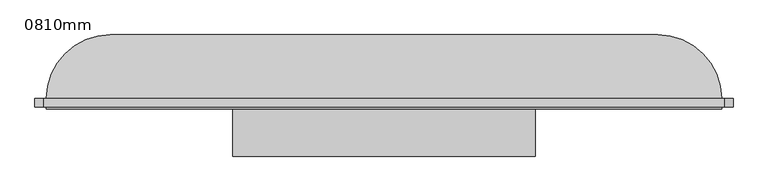
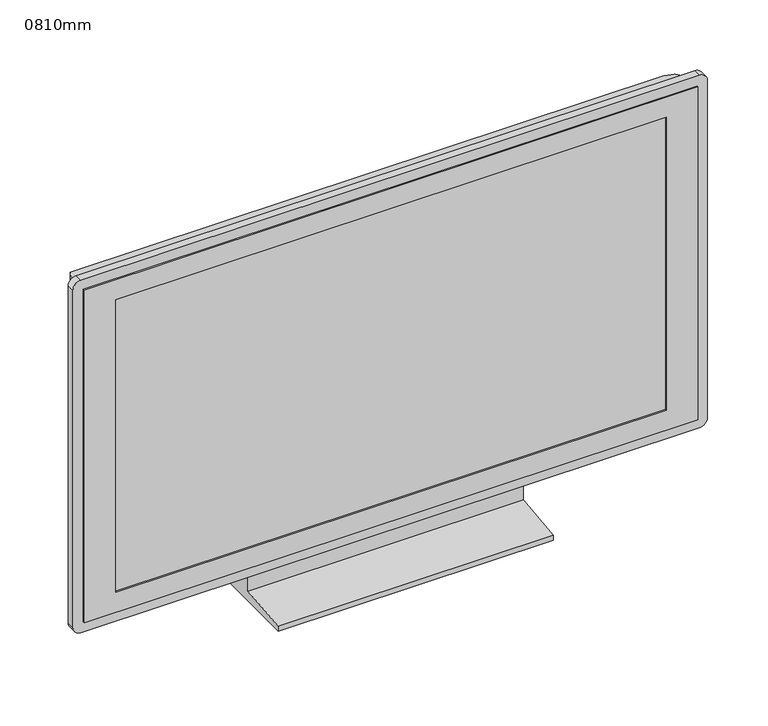
"""IFC4 building model written with IfcOpenShell, lengths in millimetres: furniture geometry, M_TV - Flat Screen : 0810mm."""

import ifcopenshell
import ifcopenshell.guid

model = None  # the IFC model being written
_history = None  # IfcOwnerHistory: only IFC2X3 demands one
_inside = {}  # id of a spatial element -> (the spatial element, [elements in it])
_under = {}  # id of a project, library or spatial element -> (it, [spatial elements below it])
_declared = {}  # id of a project -> (the project, [libraries it declares])
_typed = {}  # id of a type object -> (the type object, [elements of that type])
_made_of = {}  # id of a material, layer set ... -> (it, [elements and type objects made of it])


def new_model(schema):
    """Start an empty IFC model of exactly this schema.

    Asked for "IFC4X3", IfcOpenShell would pick the latest addendum, in which some entities
    have other attributes; the version numbers below select the first issue.
    IFC2X3 requires an IfcOwnerHistory on every rooted entity: one is made here for all.
    """
    global model, _history
    if schema == "IFC4X3":
        model = ifcopenshell.file(schema_version=(4, 3, 0, 0))
    else:
        model = ifcopenshell.file(schema=schema)
    _inside.clear()
    _under.clear()
    _declared.clear()
    _typed.clear()
    _made_of.clear()
    _history = None
    if model.schema == "IFC2X3":
        org = make("IfcOrganization", Name="unknown")
        user = make(
            "IfcPersonAndOrganization",
            ThePerson=make("IfcPerson", FamilyName="unknown"),
            TheOrganization=org,
        )
        app = make(
            "IfcApplication",
            ApplicationDeveloper=org,
            Version="unknown",
            ApplicationFullName="unknown",
            ApplicationIdentifier="unknown",
        )
        _history = make(
            "IfcOwnerHistory",
            OwningUser=user,
            OwningApplication=app,
            ChangeAction="ADDED",
            CreationDate=0,
        )
    return model


def make(cls, **values):
    """One entity of the class cls with the attributes given. An attribute that is None is left unset."""
    return model.create_entity(
        cls, **{name: value for name, value in values.items() if value is not None}
    )


def rooted(cls, **values):
    """An entity with a GlobalId (a new one), such as an element, a storey or a relation."""
    return make(cls, GlobalId=ifcopenshell.guid.new(), OwnerHistory=_history, **values)


def si_unit(unit_type, name, prefix=None):
    """IfcSIUnit, for example si_unit("LENGTHUNIT", "METRE", prefix="MILLI")."""
    return make("IfcSIUnit", UnitType=unit_type, Prefix=prefix, Name=name)


def assignment(units):
    """IfcUnitAssignment: the units of a project."""
    return None if units is None else make("IfcUnitAssignment", Units=units)


def point(xyz):
    """IfcCartesianPoint."""
    return None if xyz is None else make("IfcCartesianPoint", Coordinates=xyz)


def direction(xyz):
    """IfcDirection."""
    return None if xyz is None else make("IfcDirection", DirectionRatios=xyz)


def frame(location, z_axis=None, x_axis=None):
    """IfcAxis2Placement3D, a coordinate frame: its origin and axes. An axis left out is left unset."""
    return make(
        "IfcAxis2Placement3D",
        Location=point(location),
        Axis=direction(z_axis),
        RefDirection=direction(x_axis),
    )


def frame_2d(location, x_axis=None):
    """IfcAxis2Placement2D, a coordinate frame in the plane: its origin and x axis."""
    return make(
        "IfcAxis2Placement2D", Location=point(location), RefDirection=direction(x_axis)
    )


def origin():
    """The frame at (0, 0, 0) with its axes left unset."""
    return frame((0.0, 0.0, 0.0))


def place(relative_to, where):
    """IfcLocalPlacement: puts the frame where relative to a parent placement (None: the world)."""
    return make(
        "IfcLocalPlacement", PlacementRelTo=relative_to, RelativePlacement=where
    )


def context(
    kind, dimensions, precision=None, world=None, true_north=None, identifier=None
):
    """IfcGeometricRepresentationContext, for example the 3D "Model" context."""
    return make(
        "IfcGeometricRepresentationContext",
        ContextIdentifier=identifier,
        ContextType=kind,
        CoordinateSpaceDimension=dimensions,
        Precision=precision,
        WorldCoordinateSystem=world,
        TrueNorth=true_north,
    )


def project(units=None, contexts=None):
    """IfcProject with its units and contexts."""
    return rooted(
        "IfcProject",
        Name="project",
        RepresentationContexts=contexts,
        UnitsInContext=assignment(units),
    )


def spatial(cls, under=None, at=None, **own):
    """A site, building, storey or space (cls), placed at a placement, below another one or the project."""
    s = rooted(cls, ObjectPlacement=at, **own)
    if under is not None:
        _under.setdefault(under.id(), (under, []))[1].append(s)
    return s


def polyline(points):
    """IfcPolyline through the points."""
    return make("IfcPolyline", Points=[point(p) for p in points])


def circle_curve(where, radius):
    """IfcCircle in the frame where."""
    return make("IfcCircle", Position=where, Radius=radius)


def ellipse_curve(where, semi_axis1, semi_axis2):
    """IfcEllipse in the frame where."""
    return make(
        "IfcEllipse", Position=where, SemiAxis1=semi_axis1, SemiAxis2=semi_axis2
    )


def trimmed(basis, trim1, trim2, sense, master):
    """IfcTrimmedCurve: the piece of a basis curve between two trims."""
    return make(
        "IfcTrimmedCurve",
        BasisCurve=basis,
        Trim1=trim1,
        Trim2=trim2,
        SenseAgreement=sense,
        MasterRepresentation=master,
    )


def segment(curve, same_sense, transition):
    """IfcCompositeCurveSegment."""
    return make(
        "IfcCompositeCurveSegment",
        Transition=transition,
        SameSense=same_sense,
        ParentCurve=curve,
    )


def composite_curve(segments, self_intersect=None):
    """IfcCompositeCurve: segments joined end to end."""
    return make("IfcCompositeCurve", Segments=segments, SelfIntersect=self_intersect)


def outline(outer, holes=None, kind="AREA"):
    """IfcArbitraryClosedProfileDef: a profile drawn as a closed curve; with holes, ...WithVoids."""
    if holes is None:
        return make("IfcArbitraryClosedProfileDef", ProfileType=kind, OuterCurve=outer)
    return make(
        "IfcArbitraryProfileDefWithVoids",
        ProfileType=kind,
        OuterCurve=outer,
        InnerCurves=holes,
    )


def extrude(swept, where, along, depth):
    """IfcExtrudedAreaSolid: the profile swept, set in the frame where, extruded along a direction by depth."""
    return make(
        "IfcExtrudedAreaSolid",
        SweptArea=swept,
        Position=where,
        ExtrudedDirection=direction(along),
        Depth=depth,
    )


def faces_of(points, faces, orient=None, outer=None):
    """IfcFace entities. A face is a list of loops; a loop is a list of indices into points, from 0.

    orient and outer hold one flag for each loop. By default every Orientation is true, the
    first loop of a face is its IfcFaceOuterBound and the others are IfcFaceBound.
    """
    made = []
    for i, loops in enumerate(faces):
        bounds = []
        for j, loop in enumerate(loops):
            is_outer = j == 0 if outer is None else outer[i][j]
            bounds.append(
                make(
                    "IfcFaceOuterBound" if is_outer else "IfcFaceBound",
                    Bound=make("IfcPolyLoop", Polygon=[points[k] for k in loop]),
                    Orientation=True if orient is None else orient[i][j],
                )
            )
        made.append(make("IfcFace", Bounds=bounds))
    return made


def faceted_brep(points, faces, orient=None, outer=None, voids=None):
    """IfcFacetedBrep: a solid bounded by flat faces; with voids (closed shells), ...WithVoids."""
    shared = [point(p) for p in points]
    hull = make("IfcClosedShell", CfsFaces=faces_of(shared, faces, orient, outer))
    if voids is None:
        return make("IfcFacetedBrep", Outer=hull)
    return make(
        "IfcFacetedBrepWithVoids",
        Outer=hull,
        Voids=[
            make(cls, CfsFaces=faces_of(shared, fs, o, b)) for cls, fs, o, b in voids
        ],
    )


def shape(context_of_items, identifier, shape_type, items):
    """IfcShapeRepresentation: the items that make up one representation, for example the "Body"."""
    return make(
        "IfcShapeRepresentation",
        ContextOfItems=context_of_items,
        RepresentationIdentifier=identifier,
        RepresentationType=shape_type,
        Items=items,
    )


def source(mapping_origin, context_of_items, identifier, shape_type, items):
    """IfcRepresentationMap: a shape defined once, which mapped items show again and again."""
    return make(
        "IfcRepresentationMap",
        MappingOrigin=mapping_origin,
        MappedRepresentation=shape(context_of_items, identifier, shape_type, items),
    )


def transform(
    local_origin,
    x_axis=None,
    y_axis=None,
    z_axis=None,
    scale=None,
    scale2=None,
    scale3=None,
    uniform=True,
):
    """IfcCartesianTransformationOperator3D, or its non-uniform kind. x_axis, y_axis, z_axis: its Axis1, 2, 3."""
    if uniform:
        return make(
            "IfcCartesianTransformationOperator3D",
            Axis1=direction(x_axis),
            Axis2=direction(y_axis),
            LocalOrigin=point(local_origin),
            Scale=scale,
            Axis3=direction(z_axis),
        )
    return make(
        "IfcCartesianTransformationOperator3DnonUniform",
        Axis1=direction(x_axis),
        Axis2=direction(y_axis),
        LocalOrigin=point(local_origin),
        Scale=scale,
        Axis3=direction(z_axis),
        Scale2=scale2,
        Scale3=scale3,
    )


def mapped(mapping_source, mapping_target):
    """IfcMappedItem: shows the shape of a source again, moved by a transform."""
    return make(
        "IfcMappedItem", MappingSource=mapping_source, MappingTarget=mapping_target
    )


def made_of(thing, what):
    """Note that an element or type object is made of a material, layer set ...; save() writes the relation."""
    if what is not None:
        _made_of.setdefault(what.id(), (what, []))[1].append(thing)
    return thing


def element(
    cls,
    number,
    at=None,
    inside=None,
    cuts=None,
    type_object=None,
    material=None,
    context=None,
    identifier="Body",
    shape_type=None,
    held_by="IfcProductDefinitionShape",
    body=None,
    shapes=None,
    **own,
):
    """One element of the class cls, such as IfcWall. Its Tag is "e" and its number.

    at: its placement. inside: the storey or other place that contains it. cuts: it is an
    opening in that element (IfcRelVoidsElement). A single representation is given by context,
    identifier, shape_type and body (its items); several are given by shapes. held_by: the class
    of the entity that holds the representations. save() writes the other relations.
    """
    e = rooted(cls, Tag="e%d" % number, ObjectPlacement=at, **own)
    if body is not None:
        shapes = [shape(context, identifier, shape_type, body)]
    if shapes is not None:
        e.Representation = make(held_by, Representations=shapes)
    if inside is not None:
        _inside.setdefault(inside.id(), (inside, []))[1].append(e)
    if cuts is not None:
        rooted(
            "IfcRelVoidsElement", RelatingBuildingElement=cuts, RelatedOpeningElement=e
        )
    if type_object is not None:
        _typed.setdefault(type_object.id(), (type_object, []))[1].append(e)
    return made_of(e, material)


def aggregate(whole, parts):
    """IfcRelAggregates: a whole, such as a stair, and the parts it consists of."""
    return rooted("IfcRelAggregates", RelatingObject=whole, RelatedObjects=parts)


def save(model, path):
    """Write the relations noted so far, then the file.

    IfcRelAggregates (storeys below a building ...), IfcRelContainedInSpatialStructure (elements
    in a storey), IfcRelDefinesByType, IfcRelAssociatesMaterial and IfcRelDeclares: one each for
    every whole, place, type object, material and project.
    """
    for whole, parts in _under.values():
        aggregate(whole, parts)
    for where, things in _inside.values():
        rooted(
            "IfcRelContainedInSpatialStructure",
            RelatedElements=things,
            RelatingStructure=where,
        )
    for kind, things in _typed.values():
        rooted("IfcRelDefinesByType", RelatedObjects=things, RelatingType=kind)
    for what, things in _made_of.values():
        rooted("IfcRelAssociatesMaterial", RelatedObjects=things, RelatingMaterial=what)
    for by, libraries in _declared.values():
        rooted("IfcRelDeclares", RelatingContext=by, RelatedDefinitions=libraries)
    model.write(path)


def plane_surface(at):
    """IfcPlane: the flat surface through the origin of the frame at, square to its z axis."""
    return make("IfcPlane", Position=at)


def cylinder_surface(at, radius):
    """IfcCylindricalSurface: all points at the distance radius from the z axis of the frame at."""
    return make("IfcCylindricalSurface", Position=at, Radius=radius)


def advanced_brep(points, edges, surfaces, faces):
    """IfcAdvancedBrep: a solid bounded by faces that lie on surfaces and meet in shared edges.

    An edge is (start, end): straight between two places in points (the first is 0);
    or (start, end, curve); or (start, end, curve, False) where it runs against its curve.
    A face is (place in surfaces, loops), or (place, loops, False) where it looks against
    its surface's normal. A loop lists edges by number (the first is 1), with a minus sign
    where the edge is run from its end to its start. The first loop is the outer one.
    """
    corners = [point(p) for p in points]
    vertices = [make("IfcVertexPoint", VertexGeometry=c) for c in corners]
    made = []
    for start, end, *more in edges:
        made.append(
            make(
                "IfcEdgeCurve",
                EdgeStart=vertices[start],
                EdgeEnd=vertices[end],
                EdgeGeometry=more[0] if more else make("IfcPolyline", Points=[corners[start], corners[end]]),
                SameSense=more[1] if len(more) > 1 else True,
            )
        )
    hull = []
    for where, loops, *sense in faces:
        bounds = []
        for j, loop in enumerate(loops):
            ring = [make("IfcOrientedEdge", EdgeElement=made[abs(k) - 1], Orientation=k > 0) for k in loop]
            bounds.append(
                make(
                    "IfcFaceOuterBound" if j == 0 else "IfcFaceBound",
                    Bound=make("IfcEdgeLoop", EdgeList=ring),
                    Orientation=True,
                )
            )
        hull.append(make("IfcAdvancedFace", Bounds=bounds, FaceSurface=surfaces[where], SameSense=sense[0] if sense else True))
    return make("IfcAdvancedBrep", Outer=make("IfcClosedShell", CfsFaces=hull))


def furniture_0810mm_d9060323(model_context):
    return source(origin(), model_context, "Body", "SolidModel", [
        advanced_brep(
        [(-586.8783027, -51.4613764, 80.0), (578.9892744, -51.4613764, 80.0), (578.9892744, -51.4613764, 748.3544945), (-586.8783027, -51.4613764, 748.3544945), (468.9892744, 58.5386236, 80.0), (-476.8783027, 58.5386236, 80.0), (-476.8783027, 58.5386236, 638.3544945), (468.9892744, 58.5386236, 638.3544945)],
        [
            (0, 1),
            (1, 2),
            (2, 3),
            (3, 0),
            (4, 5),
            (5, 6),
            (6, 7),
            (7, 4),
            (0, 5, circle_curve(frame((-476.8783027, -51.4613764, 80.0), z_axis=(0.0, 0.0, -1.0), x_axis=(-1.0, 0.0, 0.0)), 110.0)),
            (4, 1, circle_curve(frame((468.9892744, -51.4613764, 80.0), z_axis=(0.0, 0.0, -1.0), x_axis=(1.0, 0.0, 0.0)), 110.0)),
            (7, 2, ellipse_curve(frame((468.9892744, -51.4613764, 638.3544945), z_axis=(0.7071067811865475, 0.0, -0.7071067811865475), x_axis=(0.7071067811865474, 0.0, 0.7071067811865476)), 155.5634919, 110.0)),
            (6, 3, ellipse_curve(frame((-476.8783027, -51.4613764, 638.3544945), z_axis=(0.7071067811865475, 0.0, 0.7071067811865476), x_axis=(-0.7071067811865476, 0.0, 0.7071067811865475)), 155.5634919, 110.0)),
        ],
        [
            plane_surface(frame((-586.8783027, -51.4613764, 748.3544945), z_axis=(0.0, -1.0, 0.0), x_axis=(-1.0, 0.0, 0.0))),
            plane_surface(frame((-586.8783027, 58.5386236, 748.3544945), z_axis=(0.0, 1.0, 0.0), x_axis=(1.0, 0.0, 0.0))),
            plane_surface(frame((-586.8783027, -51.4613764, 80.0), z_axis=(0.0, 0.0, -1.0), x_axis=(0.0, 1.0, 0.0))),
            cylinder_surface(frame((468.9892744, -51.4613764, 80.0), z_axis=(0.0, 0.0, 1.0), x_axis=(1.0, 0.0, 0.0)), 110.0),
            cylinder_surface(frame((578.9892744, -51.4613764, 638.3544945), z_axis=(-1.0, 0.0, 0.0), x_axis=(0.0, 0.0, 1.0)), 110.0),
            cylinder_surface(frame((-476.8783027, -51.4613764, 748.3544945), z_axis=(0.0, 0.0, -1.0), x_axis=(-1.0, 0.0, 0.0)), 110.0),
        ],
        [
            (0, [[1, 2, 3, 4]]),
            (1, [[5, 6, 7, 8]]),
            (2, [[-1, 9, -5, 10]]),
            (3, [[11, -2, -10, -8]]),
            (4, [[-11, -7, 12, -3]]),
            (5, [[-12, -6, -9, -4]]),
        ],
    ),
        extrude(outline(composite_curve([segment(polyline([(768.3544945, 583.9892744), (768.3544945, -591.8783027)]), True, "CONTINUOUS"), segment(trimmed(circle_curve(frame_2d((753.3544945, -591.8783027)), 15.0), [point((768.3544945, -591.8783027))], [point((753.3544945, -606.8783027))], False, "CARTESIAN"), True, "CONTINUOUS"), segment(polyline([(753.3544945, -606.8783027), (75.0, -606.8783027)]), True, "CONTINUOUS"), segment(trimmed(circle_curve(frame_2d((75.0, -591.8783027)), 15.0), [point((75.0, -606.8783027))], [point((60.0, -591.8783027))], False, "CARTESIAN"), True, "CONTINUOUS"), segment(polyline([(60.0, -591.8783027), (60.0, 583.9892744)]), True, "CONTINUOUS"), segment(trimmed(circle_curve(frame_2d((75.0, 583.9892744)), 15.0), [point((60.0, 583.9892744))], [point((75.0, 598.9892744))], False, "CARTESIAN"), True, "CONTINUOUS"), segment(polyline([(75.0, 598.9892744), (753.3544945, 598.9892744)]), True, "CONTINUOUS"), segment(trimmed(circle_curve(frame_2d((753.3544945, 583.9892744)), 15.0), [point((753.3544945, 598.9892744))], [point((768.3544945, 583.9892744))], False, "CARTESIAN"), True, "CONTINUOUS")], self_intersect=False), holes=[polyline([(748.3544945, 578.9892744), (80.0, 578.9892744), (80.0, -586.8783027), (748.3544945, -586.8783027), (748.3544945, 578.9892744)])]), frame((0.0, -66.4613764, 0.0), z_axis=(0.0, 1.0, 0.0), x_axis=(0.0, 0.0, 1.0)), (0.0, 0.0, 1.0), 15.0),
        faceted_brep([(578.9892744, -69.4613764, 748.3544945), (-586.8783027, -69.4613764, 748.3544945), (-586.8783027, -69.4613764, 80.0), (578.9892744, -69.4613764, 80.0), (-526.8783027, -69.4613764, 708.3544945), (518.9892744, -69.4613764, 708.3544945), (518.9892744, -69.4613764, 120.0), (-526.8783027, -69.4613764, 120.0), (578.9892744, -51.4613764, 748.3544945), (578.9892744, -51.4613764, 80.0), (-586.8783027, -51.4613764, 80.0), (-586.8783027, -51.4613764, 748.3544945), (-526.8783027, -66.4613764, 708.3544945), (-526.8783027, -66.4613764, 120.0), (518.9892744, -66.4613764, 120.0), (518.9892744, -66.4613764, 708.3544945)], [[[0, 1, 2, 3], [4, 5, 6, 7]], [[8, 9, 10, 11]], [[1, 0, 8, 11]], [[2, 1, 11, 10]], [[3, 2, 10, 9]], [[0, 3, 9, 8]], [[12, 13, 14, 15]], [[12, 15, 5, 4]], [[15, 14, 6, 5]], [[14, 13, 7, 6]], [[13, 12, 4, 7]]]),
        extrude(outline(polyline([(-51.4613764, 80.0), (-1.4613764, 80.0), (48.5386236, 0.0), (-151.4613764, 0.0), (-151.4613764, 10.0), (-51.4613764, 20.0), (-51.4613764, 80.0)])), frame((-265.4114084, 0.0, 0.0), z_axis=(1.0, 0.0, 0.0), x_axis=(0.0, 1.0, 0.0)), (0.0, 0.0, 1.0), 522.9337886),
    ])


if __name__ == "__main__":
    model = new_model("IFC4")
    model_context = context("Model", 3, world=origin())
    ifc_project = project(units=[si_unit("LENGTHUNIT", "METRE", prefix="MILLI")], contexts=[model_context])
    site = spatial("IfcSite", under=ifc_project)
    building = spatial("IfcBuilding", under=site)
    placement = place(None, origin())
    furniture_0810mm_shape = furniture_0810mm_d9060323(model_context)
    element("IfcFurniture", 1, ObjectType="M_TV - Flat Screen : 0810mm", at=placement, inside=building, context=model_context, shape_type="MappedRepresentation", body=[
        mapped(furniture_0810mm_shape, transform((0.0, 0.0, 0.0), x_axis=(1.0, 0.0, 0.0), y_axis=(0.0, 1.0, 0.0), z_axis=(0.0, 0.0, 1.0))),
    ])
    save(model, "model.ifc")

# Revit data of these elements
# Type "M_TV - Flat Screen : 0810mm"
#   SinAng = 0.049 cm
#   L = 104.5868 cm
#   H = 58.8354 cm
#   Thickness = 11 cm
#   Diagonal = 120 cm
#   Default Elevation = 60 cm
#   CosAng = 0.0872 cm
#   Stand [instance default] = yes
# Element 1 (IfcFurniture, "M_TV - Flat Screen : 0810mm")
#   Materials on its faces: "TV - Black", "TV - Glass", "TV - Screen"
# Materials
#   "TV - Black": class "Miscellaneous", colour RGB 49 49 49, transparency 0
#   "TV - Glass": class "Miscellaneous", colour RGB 157 157 157, transparency 0.9
#   "TV - Screen": class "Miscellaneous", colour RGB 0 0 0, transparency 0
